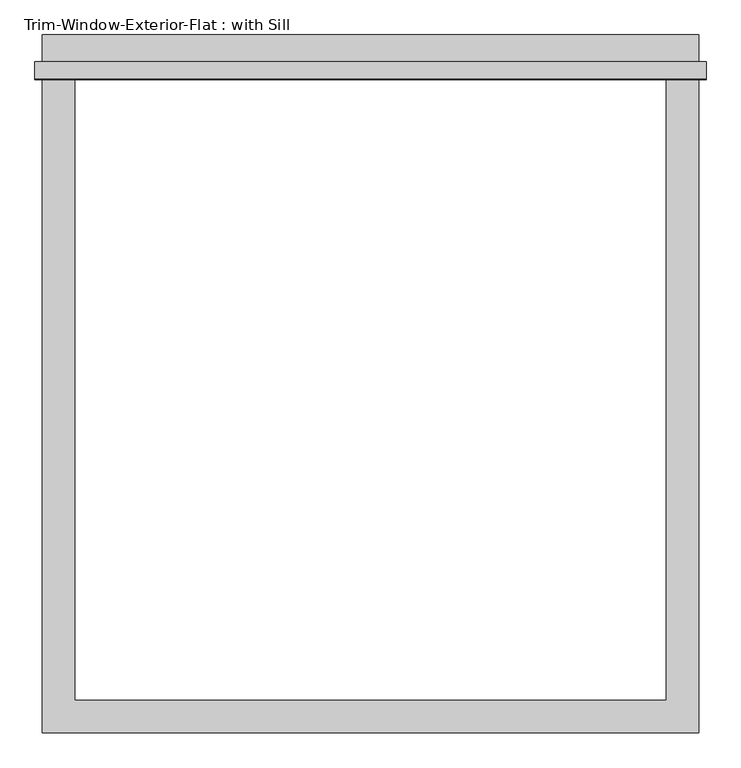
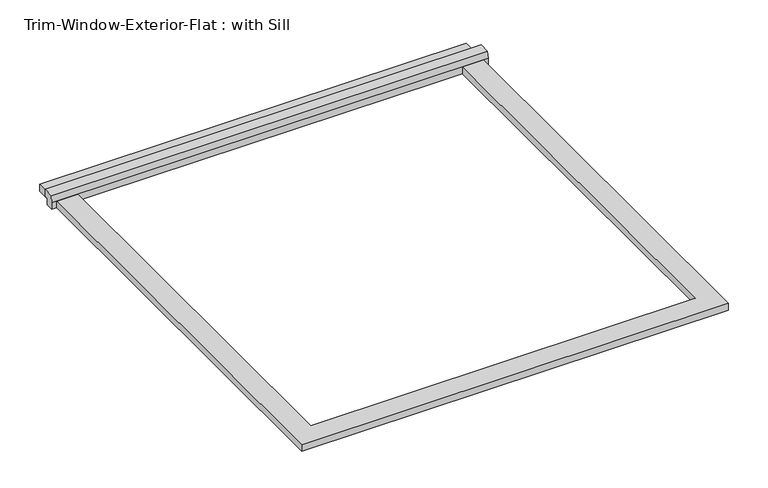
"""IFC4 building model written with IfcOpenShell, lengths in millimetres: proxy geometry, Trim-Window-Exterior-Flat : with Sill."""

import ifcopenshell
import ifcopenshell.guid

model = None  # the IFC model being written
_history = None  # IfcOwnerHistory: only IFC2X3 demands one
_inside = {}  # id of a spatial element -> (the spatial element, [elements in it])
_under = {}  # id of a project, library or spatial element -> (it, [spatial elements below it])
_declared = {}  # id of a project -> (the project, [libraries it declares])
_typed = {}  # id of a type object -> (the type object, [elements of that type])
_made_of = {}  # id of a material, layer set ... -> (it, [elements and type objects made of it])


def new_model(schema):
    """Start an empty IFC model of exactly this schema.

    Asked for "IFC4X3", IfcOpenShell would pick the latest addendum, in which some entities
    have other attributes; the version numbers below select the first issue.
    IFC2X3 requires an IfcOwnerHistory on every rooted entity: one is made here for all.
    """
    global model, _history
    if schema == "IFC4X3":
        model = ifcopenshell.file(schema_version=(4, 3, 0, 0))
    else:
        model = ifcopenshell.file(schema=schema)
    _inside.clear()
    _under.clear()
    _declared.clear()
    _typed.clear()
    _made_of.clear()
    _history = None
    if model.schema == "IFC2X3":
        org = make("IfcOrganization", Name="unknown")
        user = make(
            "IfcPersonAndOrganization",
            ThePerson=make("IfcPerson", FamilyName="unknown"),
            TheOrganization=org,
        )
        app = make(
            "IfcApplication",
            ApplicationDeveloper=org,
            Version="unknown",
            ApplicationFullName="unknown",
            ApplicationIdentifier="unknown",
        )
        _history = make(
            "IfcOwnerHistory",
            OwningUser=user,
            OwningApplication=app,
            ChangeAction="ADDED",
            CreationDate=0,
        )
    return model


def make(cls, **values):
    """One entity of the class cls with the attributes given. An attribute that is None is left unset."""
    return model.create_entity(
        cls, **{name: value for name, value in values.items() if value is not None}
    )


def rooted(cls, **values):
    """An entity with a GlobalId (a new one), such as an element, a storey or a relation."""
    return make(cls, GlobalId=ifcopenshell.guid.new(), OwnerHistory=_history, **values)


def si_unit(unit_type, name, prefix=None):
    """IfcSIUnit, for example si_unit("LENGTHUNIT", "METRE", prefix="MILLI")."""
    return make("IfcSIUnit", UnitType=unit_type, Prefix=prefix, Name=name)


def assignment(units):
    """IfcUnitAssignment: the units of a project."""
    return None if units is None else make("IfcUnitAssignment", Units=units)


def point(xyz):
    """IfcCartesianPoint."""
    return None if xyz is None else make("IfcCartesianPoint", Coordinates=xyz)


def direction(xyz):
    """IfcDirection."""
    return None if xyz is None else make("IfcDirection", DirectionRatios=xyz)


def frame(location, z_axis=None, x_axis=None):
    """IfcAxis2Placement3D, a coordinate frame: its origin and axes. An axis left out is left unset."""
    return make(
        "IfcAxis2Placement3D",
        Location=point(location),
        Axis=direction(z_axis),
        RefDirection=direction(x_axis),
    )


def origin():
    """The frame at (0, 0, 0) with its axes left unset."""
    return frame((0.0, 0.0, 0.0))


def origin_with_axes():
    """The frame at (0, 0, 0) with the z axis (0, 0, 1) and the x axis (1, 0, 0) written out."""
    return frame((0.0, 0.0, 0.0), z_axis=(0.0, 0.0, 1.0), x_axis=(1.0, 0.0, 0.0))


def place(relative_to, where):
    """IfcLocalPlacement: puts the frame where relative to a parent placement (None: the world)."""
    return make(
        "IfcLocalPlacement", PlacementRelTo=relative_to, RelativePlacement=where
    )


def context(
    kind, dimensions, precision=None, world=None, true_north=None, identifier=None
):
    """IfcGeometricRepresentationContext, for example the 3D "Model" context."""
    return make(
        "IfcGeometricRepresentationContext",
        ContextIdentifier=identifier,
        ContextType=kind,
        CoordinateSpaceDimension=dimensions,
        Precision=precision,
        WorldCoordinateSystem=world,
        TrueNorth=true_north,
    )


def project(units=None, contexts=None):
    """IfcProject with its units and contexts."""
    return rooted(
        "IfcProject",
        Name="project",
        RepresentationContexts=contexts,
        UnitsInContext=assignment(units),
    )


def spatial(cls, under=None, at=None, **own):
    """A site, building, storey or space (cls), placed at a placement, below another one or the project."""
    s = rooted(cls, ObjectPlacement=at, **own)
    if under is not None:
        _under.setdefault(under.id(), (under, []))[1].append(s)
    return s


def polyline(points):
    """IfcPolyline through the points."""
    return make("IfcPolyline", Points=[point(p) for p in points])


def outline(outer, holes=None, kind="AREA"):
    """IfcArbitraryClosedProfileDef: a profile drawn as a closed curve; with holes, ...WithVoids."""
    if holes is None:
        return make("IfcArbitraryClosedProfileDef", ProfileType=kind, OuterCurve=outer)
    return make(
        "IfcArbitraryProfileDefWithVoids",
        ProfileType=kind,
        OuterCurve=outer,
        InnerCurves=holes,
    )


def extrude(swept, where, along, depth):
    """IfcExtrudedAreaSolid: the profile swept, set in the frame where, extruded along a direction by depth."""
    return make(
        "IfcExtrudedAreaSolid",
        SweptArea=swept,
        Position=where,
        ExtrudedDirection=direction(along),
        Depth=depth,
    )


def shape(context_of_items, identifier, shape_type, items):
    """IfcShapeRepresentation: the items that make up one representation, for example the "Body"."""
    return make(
        "IfcShapeRepresentation",
        ContextOfItems=context_of_items,
        RepresentationIdentifier=identifier,
        RepresentationType=shape_type,
        Items=items,
    )


def source(mapping_origin, context_of_items, identifier, shape_type, items):
    """IfcRepresentationMap: a shape defined once, which mapped items show again and again."""
    return make(
        "IfcRepresentationMap",
        MappingOrigin=mapping_origin,
        MappedRepresentation=shape(context_of_items, identifier, shape_type, items),
    )


def transform(
    local_origin,
    x_axis=None,
    y_axis=None,
    z_axis=None,
    scale=None,
    scale2=None,
    scale3=None,
    uniform=True,
):
    """IfcCartesianTransformationOperator3D, or its non-uniform kind. x_axis, y_axis, z_axis: its Axis1, 2, 3."""
    if uniform:
        return make(
            "IfcCartesianTransformationOperator3D",
            Axis1=direction(x_axis),
            Axis2=direction(y_axis),
            LocalOrigin=point(local_origin),
            Scale=scale,
            Axis3=direction(z_axis),
        )
    return make(
        "IfcCartesianTransformationOperator3DnonUniform",
        Axis1=direction(x_axis),
        Axis2=direction(y_axis),
        LocalOrigin=point(local_origin),
        Scale=scale,
        Axis3=direction(z_axis),
        Scale2=scale2,
        Scale3=scale3,
    )


def mapped(mapping_source, mapping_target):
    """IfcMappedItem: shows the shape of a source again, moved by a transform."""
    return make(
        "IfcMappedItem", MappingSource=mapping_source, MappingTarget=mapping_target
    )


def made_of(thing, what):
    """Note that an element or type object is made of a material, layer set ...; save() writes the relation."""
    if what is not None:
        _made_of.setdefault(what.id(), (what, []))[1].append(thing)
    return thing


def element(
    cls,
    number,
    at=None,
    inside=None,
    cuts=None,
    type_object=None,
    material=None,
    context=None,
    identifier="Body",
    shape_type=None,
    held_by="IfcProductDefinitionShape",
    body=None,
    shapes=None,
    **own,
):
    """One element of the class cls, such as IfcWall. Its Tag is "e" and its number.

    at: its placement. inside: the storey or other place that contains it. cuts: it is an
    opening in that element (IfcRelVoidsElement). A single representation is given by context,
    identifier, shape_type and body (its items); several are given by shapes. held_by: the class
    of the entity that holds the representations. save() writes the other relations.
    """
    e = rooted(cls, Tag="e%d" % number, ObjectPlacement=at, **own)
    if body is not None:
        shapes = [shape(context, identifier, shape_type, body)]
    if shapes is not None:
        e.Representation = make(held_by, Representations=shapes)
    if inside is not None:
        _inside.setdefault(inside.id(), (inside, []))[1].append(e)
    if cuts is not None:
        rooted(
            "IfcRelVoidsElement", RelatingBuildingElement=cuts, RelatedOpeningElement=e
        )
    if type_object is not None:
        _typed.setdefault(type_object.id(), (type_object, []))[1].append(e)
    return made_of(e, material)


def aggregate(whole, parts):
    """IfcRelAggregates: a whole, such as a stair, and the parts it consists of."""
    return rooted("IfcRelAggregates", RelatingObject=whole, RelatedObjects=parts)


def save(model, path):
    """Write the relations noted so far, then the file.

    IfcRelAggregates (storeys below a building ...), IfcRelContainedInSpatialStructure (elements
    in a storey), IfcRelDefinesByType, IfcRelAssociatesMaterial and IfcRelDeclares: one each for
    every whole, place, type object, material and project.
    """
    for whole, parts in _under.values():
        aggregate(whole, parts)
    for where, things in _inside.values():
        rooted(
            "IfcRelContainedInSpatialStructure",
            RelatedElements=things,
            RelatingStructure=where,
        )
    for kind, things in _typed.values():
        rooted("IfcRelDefinesByType", RelatedObjects=things, RelatingType=kind)
    for what, things in _made_of.values():
        rooted("IfcRelAssociatesMaterial", RelatedObjects=things, RelatingMaterial=what)
    for by, libraries in _declared.values():
        rooted("IfcRelDeclares", RelatingContext=by, RelatedDefinitions=libraries)
    model.write(path)


def trim_window_exterior_flat_with_sill_26b0c1ac(model_context):
    return source(origin(), model_context, "Body", "SweptSolid", [
        extrude(outline(polyline([(577.85, 1114.3823709), (-577.85, 1114.3823709), (-577.85, 1171.5323709), (577.85, 1171.5323709), (577.85, 1114.3823709)])), origin_with_axes(), (0.0, 0.0, 1.0), 19.05),
        extrude(outline(polyline([(1123.95, 38.1), (1123.95, 19.05), (1114.3823709, 19.05), (1114.3823709, 0.0), (1092.2, 0.0), (1092.2, 19.05), (1094.6580645, 38.1), (1123.95, 38.1)])), frame((-590.55, 0.0, 0.0), z_axis=(1.0, 0.0, 0.0), x_axis=(0.0, 1.0, 0.0)), (0.0, 0.0, 1.0), 1181.1),
        extrude(outline(polyline([(-577.85, -57.15), (-577.85, 1092.2), (-520.7, 1092.2), (-520.7, 0.0), (520.7, 0.0), (520.7, 1092.2), (577.85, 1092.2), (577.85, -57.15), (-577.85, -57.15)])), origin_with_axes(), (0.0, 0.0, 1.0), 19.05),
    ])


if __name__ == "__main__":
    model = new_model("IFC4")
    model_context = context("Model", 3, world=origin())
    ifc_project = project(units=[si_unit("LENGTHUNIT", "METRE", prefix="MILLI")], contexts=[model_context])
    site = spatial("IfcSite", under=ifc_project)
    building = spatial("IfcBuilding", under=site)
    placement = place(None, origin())
    trim_window_exterior_flat_with_sill_shape = trim_window_exterior_flat_with_sill_26b0c1ac(model_context)
    element("IfcBuildingElementProxy", 1, Name="Trim-Window-Exterior-Flat : with Sill", ObjectType="Trim-Window-Exterior-Flat : with Sill", at=placement, inside=building, context=model_context, shape_type="MappedRepresentation", body=[
        mapped(trim_window_exterior_flat_with_sill_shape, transform((0.0, 0.0, 0.0), x_axis=(1.0, 0.0, 0.0), y_axis=(0.0, 1.0, 0.0), z_axis=(0.0, 0.0, 1.0))),
    ])
    save(model, "model.ifc")

# Revit data of these elements
# Type "Trim-Window-Exterior-Flat : with Sill"
#   Trim Width = 0' - 2 1/4"
#   Trim Thickness_Picture Frame = 0' - 1 1/4"
#   Trim Thickness_with Sill = 0' - 0 3/4"
#   Sill Thickness = 0' - 1 1/4"
#   Opening Width [instance default] = 2' - 0"
#   Opening Height [instance default] = 3' - 0"
#   Default Elevation = 4' - 0"
#   Sill = yes
#   Picture Frame = no
#   Trim Material [instance default] = none
# Element 1 (IfcBuildingElementProxy, "Trim-Window-Exterior-Flat : with Sill")
#   Opening Width = 3' - 5"
#   Opening Height = 3' - 7"
#   Trim Material = Clad - White
#   Materials on its faces: "Clad - White"
# Materials
#   "Clad - White": class "Wood", colour RGB 242 242 238, transparency 0, Cost = 0
